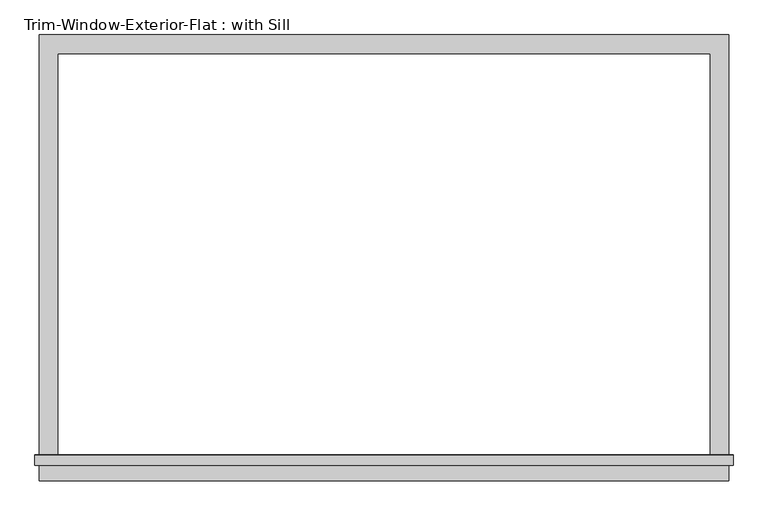
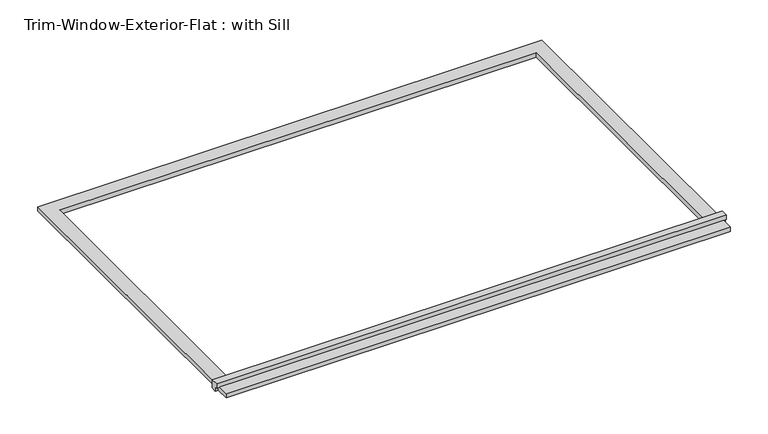
"""IFC4 building model written with IfcOpenShell, lengths in millimetres: proxy geometry, Trim-Window-Exterior-Flat : with Sill."""

import ifcopenshell
import ifcopenshell.guid

model = None  # the IFC model being written
_history = None  # IfcOwnerHistory: only IFC2X3 demands one
_inside = {}  # id of a spatial element -> (the spatial element, [elements in it])
_under = {}  # id of a project, library or spatial element -> (it, [spatial elements below it])
_declared = {}  # id of a project -> (the project, [libraries it declares])
_typed = {}  # id of a type object -> (the type object, [elements of that type])
_made_of = {}  # id of a material, layer set ... -> (it, [elements and type objects made of it])


def new_model(schema):
    """Start an empty IFC model of exactly this schema.

    Asked for "IFC4X3", IfcOpenShell would pick the latest addendum, in which some entities
    have other attributes; the version numbers below select the first issue.
    IFC2X3 requires an IfcOwnerHistory on every rooted entity: one is made here for all.
    """
    global model, _history
    if schema == "IFC4X3":
        model = ifcopenshell.file(schema_version=(4, 3, 0, 0))
    else:
        model = ifcopenshell.file(schema=schema)
    _inside.clear()
    _under.clear()
    _declared.clear()
    _typed.clear()
    _made_of.clear()
    _history = None
    if model.schema == "IFC2X3":
        org = make("IfcOrganization", Name="unknown")
        user = make(
            "IfcPersonAndOrganization",
            ThePerson=make("IfcPerson", FamilyName="unknown"),
            TheOrganization=org,
        )
        app = make(
            "IfcApplication",
            ApplicationDeveloper=org,
            Version="unknown",
            ApplicationFullName="unknown",
            ApplicationIdentifier="unknown",
        )
        _history = make(
            "IfcOwnerHistory",
            OwningUser=user,
            OwningApplication=app,
            ChangeAction="ADDED",
            CreationDate=0,
        )
    return model


def make(cls, **values):
    """One entity of the class cls with the attributes given. An attribute that is None is left unset."""
    return model.create_entity(
        cls, **{name: value for name, value in values.items() if value is not None}
    )


def rooted(cls, **values):
    """An entity with a GlobalId (a new one), such as an element, a storey or a relation."""
    return make(cls, GlobalId=ifcopenshell.guid.new(), OwnerHistory=_history, **values)


def si_unit(unit_type, name, prefix=None):
    """IfcSIUnit, for example si_unit("LENGTHUNIT", "METRE", prefix="MILLI")."""
    return make("IfcSIUnit", UnitType=unit_type, Prefix=prefix, Name=name)


def assignment(units):
    """IfcUnitAssignment: the units of a project."""
    return None if units is None else make("IfcUnitAssignment", Units=units)


def point(xyz):
    """IfcCartesianPoint."""
    return None if xyz is None else make("IfcCartesianPoint", Coordinates=xyz)


def direction(xyz):
    """IfcDirection."""
    return None if xyz is None else make("IfcDirection", DirectionRatios=xyz)


def frame(location, z_axis=None, x_axis=None):
    """IfcAxis2Placement3D, a coordinate frame: its origin and axes. An axis left out is left unset."""
    return make(
        "IfcAxis2Placement3D",
        Location=point(location),
        Axis=direction(z_axis),
        RefDirection=direction(x_axis),
    )


def origin():
    """The frame at (0, 0, 0) with its axes left unset."""
    return frame((0.0, 0.0, 0.0))


def origin_with_axes():
    """The frame at (0, 0, 0) with the z axis (0, 0, 1) and the x axis (1, 0, 0) written out."""
    return frame((0.0, 0.0, 0.0), z_axis=(0.0, 0.0, 1.0), x_axis=(1.0, 0.0, 0.0))


def place(relative_to, where):
    """IfcLocalPlacement: puts the frame where relative to a parent placement (None: the world)."""
    return make(
        "IfcLocalPlacement", PlacementRelTo=relative_to, RelativePlacement=where
    )


def context(
    kind, dimensions, precision=None, world=None, true_north=None, identifier=None
):
    """IfcGeometricRepresentationContext, for example the 3D "Model" context."""
    return make(
        "IfcGeometricRepresentationContext",
        ContextIdentifier=identifier,
        ContextType=kind,
        CoordinateSpaceDimension=dimensions,
        Precision=precision,
        WorldCoordinateSystem=world,
        TrueNorth=true_north,
    )


def project(units=None, contexts=None):
    """IfcProject with its units and contexts."""
    return rooted(
        "IfcProject",
        Name="project",
        RepresentationContexts=contexts,
        UnitsInContext=assignment(units),
    )


def spatial(cls, under=None, at=None, **own):
    """A site, building, storey or space (cls), placed at a placement, below another one or the project."""
    s = rooted(cls, ObjectPlacement=at, **own)
    if under is not None:
        _under.setdefault(under.id(), (under, []))[1].append(s)
    return s


def polyline(points):
    """IfcPolyline through the points."""
    return make("IfcPolyline", Points=[point(p) for p in points])


def outline(outer, holes=None, kind="AREA"):
    """IfcArbitraryClosedProfileDef: a profile drawn as a closed curve; with holes, ...WithVoids."""
    if holes is None:
        return make("IfcArbitraryClosedProfileDef", ProfileType=kind, OuterCurve=outer)
    return make(
        "IfcArbitraryProfileDefWithVoids",
        ProfileType=kind,
        OuterCurve=outer,
        InnerCurves=holes,
    )


def extrude(swept, where, along, depth):
    """IfcExtrudedAreaSolid: the profile swept, set in the frame where, extruded along a direction by depth."""
    return make(
        "IfcExtrudedAreaSolid",
        SweptArea=swept,
        Position=where,
        ExtrudedDirection=direction(along),
        Depth=depth,
    )


def shape(context_of_items, identifier, shape_type, items):
    """IfcShapeRepresentation: the items that make up one representation, for example the "Body"."""
    return make(
        "IfcShapeRepresentation",
        ContextOfItems=context_of_items,
        RepresentationIdentifier=identifier,
        RepresentationType=shape_type,
        Items=items,
    )


def source(mapping_origin, context_of_items, identifier, shape_type, items):
    """IfcRepresentationMap: a shape defined once, which mapped items show again and again."""
    return make(
        "IfcRepresentationMap",
        MappingOrigin=mapping_origin,
        MappedRepresentation=shape(context_of_items, identifier, shape_type, items),
    )


def transform(
    local_origin,
    x_axis=None,
    y_axis=None,
    z_axis=None,
    scale=None,
    scale2=None,
    scale3=None,
    uniform=True,
):
    """IfcCartesianTransformationOperator3D, or its non-uniform kind. x_axis, y_axis, z_axis: its Axis1, 2, 3."""
    if uniform:
        return make(
            "IfcCartesianTransformationOperator3D",
            Axis1=direction(x_axis),
            Axis2=direction(y_axis),
            LocalOrigin=point(local_origin),
            Scale=scale,
            Axis3=direction(z_axis),
        )
    return make(
        "IfcCartesianTransformationOperator3DnonUniform",
        Axis1=direction(x_axis),
        Axis2=direction(y_axis),
        LocalOrigin=point(local_origin),
        Scale=scale,
        Axis3=direction(z_axis),
        Scale2=scale2,
        Scale3=scale3,
    )


def mapped(mapping_source, mapping_target):
    """IfcMappedItem: shows the shape of a source again, moved by a transform."""
    return make(
        "IfcMappedItem", MappingSource=mapping_source, MappingTarget=mapping_target
    )


def made_of(thing, what):
    """Note that an element or type object is made of a material, layer set ...; save() writes the relation."""
    if what is not None:
        _made_of.setdefault(what.id(), (what, []))[1].append(thing)
    return thing


def element(
    cls,
    number,
    at=None,
    inside=None,
    cuts=None,
    type_object=None,
    material=None,
    context=None,
    identifier="Body",
    shape_type=None,
    held_by="IfcProductDefinitionShape",
    body=None,
    shapes=None,
    **own,
):
    """One element of the class cls, such as IfcWall. Its Tag is "e" and its number.

    at: its placement. inside: the storey or other place that contains it. cuts: it is an
    opening in that element (IfcRelVoidsElement). A single representation is given by context,
    identifier, shape_type and body (its items); several are given by shapes. held_by: the class
    of the entity that holds the representations. save() writes the other relations.
    """
    e = rooted(cls, Tag="e%d" % number, ObjectPlacement=at, **own)
    if body is not None:
        shapes = [shape(context, identifier, shape_type, body)]
    if shapes is not None:
        e.Representation = make(held_by, Representations=shapes)
    if inside is not None:
        _inside.setdefault(inside.id(), (inside, []))[1].append(e)
    if cuts is not None:
        rooted(
            "IfcRelVoidsElement", RelatingBuildingElement=cuts, RelatedOpeningElement=e
        )
    if type_object is not None:
        _typed.setdefault(type_object.id(), (type_object, []))[1].append(e)
    return made_of(e, material)


def aggregate(whole, parts):
    """IfcRelAggregates: a whole, such as a stair, and the parts it consists of."""
    return rooted("IfcRelAggregates", RelatingObject=whole, RelatedObjects=parts)


def save(model, path):
    """Write the relations noted so far, then the file.

    IfcRelAggregates (storeys below a building ...), IfcRelContainedInSpatialStructure (elements
    in a storey), IfcRelDefinesByType, IfcRelAssociatesMaterial and IfcRelDeclares: one each for
    every whole, place, type object, material and project.
    """
    for whole, parts in _under.values():
        aggregate(whole, parts)
    for where, things in _inside.values():
        rooted(
            "IfcRelContainedInSpatialStructure",
            RelatedElements=things,
            RelatingStructure=where,
        )
    for kind, things in _typed.values():
        rooted("IfcRelDefinesByType", RelatedObjects=things, RelatingType=kind)
    for what, things in _made_of.values():
        rooted("IfcRelAssociatesMaterial", RelatedObjects=things, RelatingMaterial=what)
    for by, libraries in _declared.values():
        rooted("IfcRelDeclares", RelatingContext=by, RelatedDefinitions=libraries)
    model.write(path)


def trim_window_exterior_flat_with_sill_97a7de1c(model_context):
    return source(origin(), model_context, "Body", "SweptSolid", [
        extrude(outline(polyline([(1047.75, -1241.3823709), (1047.75, -1298.5323709), (-1047.75, -1298.5323709), (-1047.75, -1241.3823709), (1047.75, -1241.3823709)])), origin_with_axes(), (0.0, 0.0, 1.0), 19.05),
        extrude(outline(polyline([(-1250.95, 38.1), (-1221.6580645, 38.1), (-1219.2, 19.05), (-1219.2, 0.0), (-1241.3823709, 0.0), (-1241.3823709, 19.05), (-1250.95, 19.05), (-1250.95, 38.1)])), frame((-1060.45, 0.0, 0.0), z_axis=(1.0, 0.0, 0.0), x_axis=(0.0, 1.0, 0.0)), (0.0, 0.0, 1.0), 2120.9),
        extrude(outline(polyline([(-1047.75, 57.15), (1047.75, 57.15), (1047.75, -1219.2), (990.6, -1219.2), (990.6, 0.0), (-990.6, 0.0), (-990.6, -1219.2), (-1047.75, -1219.2), (-1047.75, 57.15)])), origin_with_axes(), (0.0, 0.0, 1.0), 19.05),
    ])


if __name__ == "__main__":
    model = new_model("IFC4")
    model_context = context("Model", 3, world=origin())
    ifc_project = project(units=[si_unit("LENGTHUNIT", "METRE", prefix="MILLI")], contexts=[model_context])
    site = spatial("IfcSite", under=ifc_project)
    building = spatial("IfcBuilding", under=site)
    placement = place(None, origin())
    trim_window_exterior_flat_with_sill_shape = trim_window_exterior_flat_with_sill_97a7de1c(model_context)
    element("IfcBuildingElementProxy", 1, Name="Trim-Window-Exterior-Flat : with Sill", ObjectType="Trim-Window-Exterior-Flat : with Sill", at=placement, inside=building, context=model_context, shape_type="MappedRepresentation", body=[
        mapped(trim_window_exterior_flat_with_sill_shape, transform((0.0, 0.0, 0.0), x_axis=(1.0, 0.0, 0.0), y_axis=(0.0, 1.0, 0.0), z_axis=(0.0, 0.0, 1.0))),
    ])
    save(model, "model.ifc")

# Revit data of these elements
# Type "Trim-Window-Exterior-Flat : with Sill"
#   Trim Width = 0' - 2 1/4"
#   Trim Thickness_Picture Frame = 0' - 1 1/4"
#   Trim Thickness_with Sill = 0' - 0 3/4"
#   Sill Thickness = 0' - 1 1/4"
#   Opening Width [instance default] = 2' - 0"
#   Opening Height [instance default] = 3' - 0"
#   Default Elevation = 4' - 0"
#   Sill = yes
#   Picture Frame = no
#   Trim Material [instance default] = none
# Element 1 (IfcBuildingElementProxy, "Trim-Window-Exterior-Flat : with Sill")
#   Opening Width = 6' - 6"
#   Opening Height = 4' - 0"
#   Trim Material = Clad - White
#   Materials on its faces: "Clad - White"
# Materials
#   "Clad - White": class "Wood", colour RGB 242 242 238, transparency 0, Cost = 0
